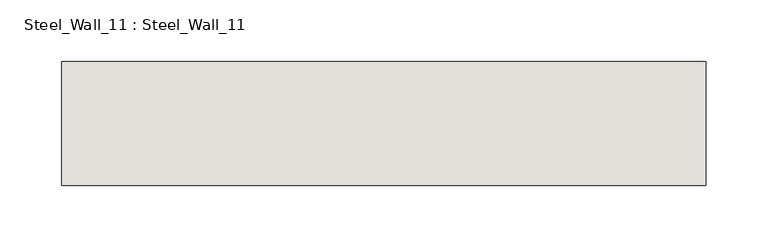
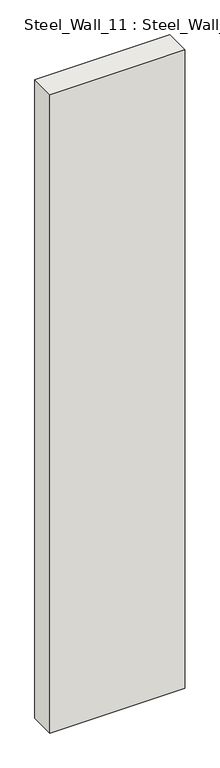
"""IFC4 building model written with IfcOpenShell, lengths in millimetres: wall geometry, Steel_Wall_11 : Steel_Wall_11."""

from ifc_helpers import new_model, si_unit, frame, origin, place, context, project, spatial, polyline, outline, extrude, source, transform, mapped, element, save


def steel_wall_11_steel_wall_11_b2c771ff(model_context):
    return source(origin(), model_context, "Body", "SweptSolid", [
        extrude(outline(polyline([(4785.0, 7415.0), (4265.0, 7415.0), (4265.0, 7515.0), (4785.0, 7515.0), (4785.0, 7415.0)])), frame((0.0, 0.0, 250.0), z_axis=(0.0, 0.0, 1.0), x_axis=(1.0, 0.0, 0.0)), (0.0, 0.0, 1.0), 2600.0),
    ])


if __name__ == "__main__":
    model = new_model("IFC4")
    model_context = context("Model", 3, world=origin())
    ifc_project = project(units=[si_unit("LENGTHUNIT", "METRE", prefix="MILLI")], contexts=[model_context])
    site = spatial("IfcSite", under=ifc_project)
    building = spatial("IfcBuilding", under=site)
    placement = place(None, origin())
    steel_wall_11_steel_wall_11_shape = steel_wall_11_steel_wall_11_b2c771ff(model_context)
    element("IfcWall", 1, ObjectType="Steel_Wall_11 : Steel_Wall_11", at=placement, inside=building, context=model_context, shape_type="MappedRepresentation", body=[
        mapped(steel_wall_11_steel_wall_11_shape, transform((0.0, 0.0, 0.0), x_axis=(1.0, 0.0, 0.0), y_axis=(0.0, 1.0, 0.0), z_axis=(0.0, 0.0, 1.0))),
    ])
    save(model, "model.ifc")

# Revit data of these elements
# Type "Steel_Wall_11 : Steel_Wall_11"
#   NameOverride = "Steel_Wall_11"
# Element 1 (IfcWall, "Steel_Wall_11 : Steel_Wall_11")
#   Materials on its faces: "IfcSurfaceStyle #33"
# Materials
#   "IfcSurfaceStyle #33": class "Unassigned", colour RGB 214 214 214, transparency 0
